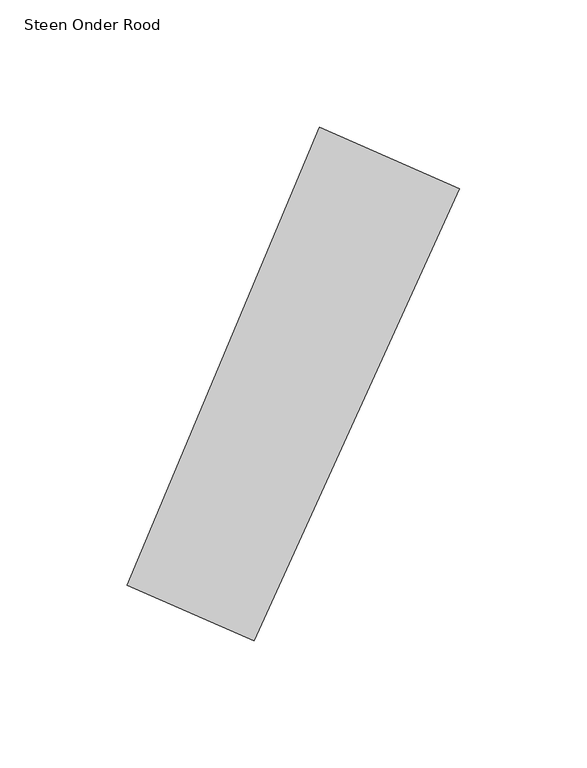
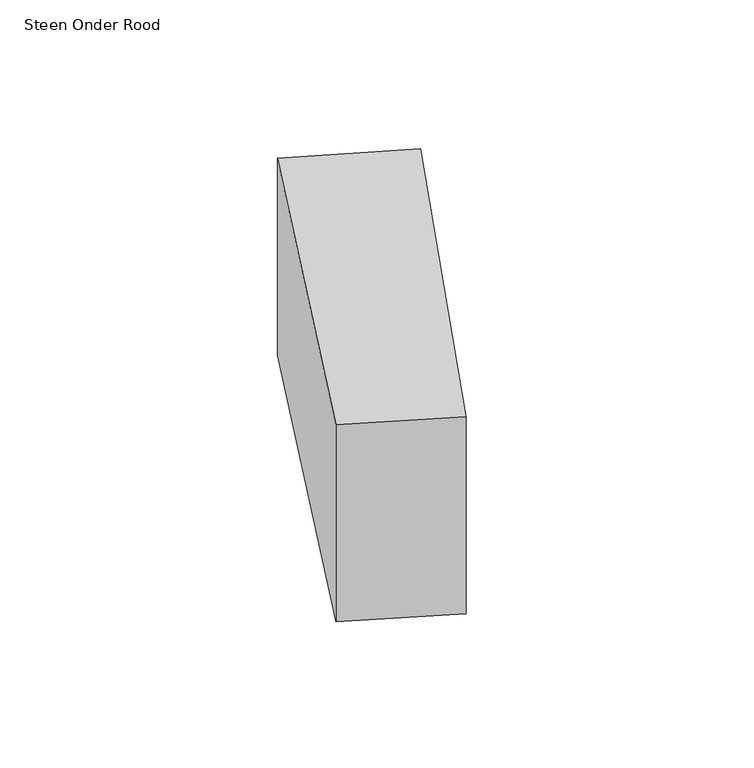
"""IFC4 building model written with IfcOpenShell, lengths in millimetres: proxy geometry, 00_GMA_steen_versie_4 : Steen Onder Rood."""

from ifc_helpers import new_model, si_unit, origin, origin_with_axes, place, context, project, spatial, polyline, outline, extrude, source, transform, mapped, element, save


def steen_onder_rood_0ac48f07(model_context):
    return source(origin(), model_context, "Body", "SweptSolid", [
        extrude(outline(polyline([(140.3520431, 157.0676512), (59.5216401, -20.4141133), (9.7745444, 1.3700991), (85.3836019, 181.1382865), (140.3520431, 157.0676512)])), origin_with_axes(), (0.0, 0.0, 1.0), 100.0),
    ])


if __name__ == "__main__":
    model = new_model("IFC4")
    model_context = context("Model", 3, world=origin())
    ifc_project = project(units=[si_unit("LENGTHUNIT", "METRE", prefix="MILLI")], contexts=[model_context])
    site = spatial("IfcSite", under=ifc_project)
    building = spatial("IfcBuilding", under=site)
    placement = place(None, origin())
    steen_onder_rood_shape = steen_onder_rood_0ac48f07(model_context)
    element("IfcBuildingElementProxy", 1, Name="00_GMA_steen_versie_4 : Steen Onder Rood", ObjectType="00_GMA_steen_versie_4 : Steen Onder Rood", at=placement, inside=building, context=model_context, shape_type="MappedRepresentation", body=[
        mapped(steen_onder_rood_shape, transform((0.0, 0.0, 0.0), x_axis=(1.0, 0.0, 0.0), y_axis=(0.0, 1.0, 0.0), z_axis=(0.0, 0.0, 1.0))),
    ])
    save(model, "model.ifc")

# Revit data of these elements
# Type "00_GMA_steen_versie_4 : Steen Onder Rood"
#   StootVoegHalfBoven [instance default] = 5 mm
#   StootVoegHalf [instance default] = 5 mm
#   StootVoegBreedteOnder = 10 mm
#   StootVoegBreedteBoven = 10 mm
#   Steendikte = 100 mm
#   LintVoegOnderHalf = 0 mm
#   LintVoegOnder = 0 mm
#   LintVoegBovenHalf = 5 mm
#   LintVoegBoven = 10 mm
#   materiaal = 21_steen_rood
#   MateriaalVoeg = none
#   Default Elevation = 0
# Element 1 (IfcBuildingElementProxy, "00_GMA_steen_versie_4 : Steen Onder Rood")
#   Materials on its faces: "21_steen_rood"
# Materials
#   "21_steen_rood": class "Unassigned", colour RGB 213 111 43, transparency 0, Cost = 0
